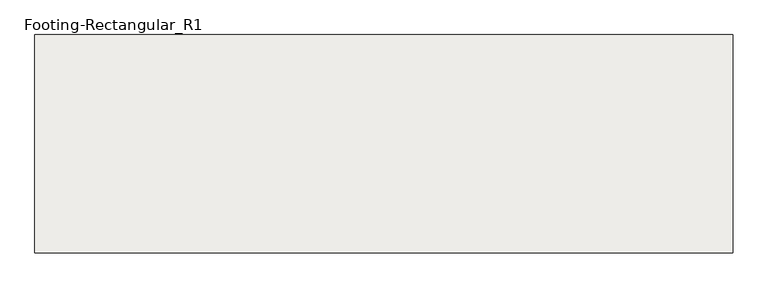
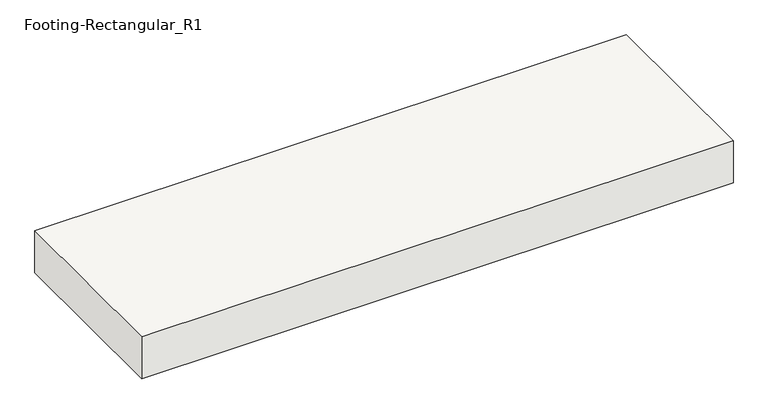
"""IFC4 building model written with IfcOpenShell, lengths in millimetres: slab geometry, Footing-Rectangular_R1 : H_SF_AR_S18_W8000xL2500xT500_Bitumen_F5."""

from ifc_helpers import new_model, si_unit, frame, origin, place, context, project, spatial, polyline, outline, extrude, source, transform, mapped, element, save


def footing_rectangular_r1_282b4f06(model_context):
    return source(origin(), model_context, "Body", "SweptSolid", [
        extrude(outline(polyline([(4000.0, 1250.0), (4000.0, -1250.0), (-4000.0, -1250.0), (-4000.0, 1250.0), (4000.0, 1250.0)])), frame((0.0, 0.0, -600.0), z_axis=(0.0, 0.0, 1.0), x_axis=(1.0, 0.0, 0.0)), (0.0, 0.0, 1.0), 600.0),
    ])


if __name__ == "__main__":
    model = new_model("IFC4")
    model_context = context("Model", 3, world=origin())
    ifc_project = project(units=[si_unit("LENGTHUNIT", "METRE", prefix="MILLI")], contexts=[model_context])
    site = spatial("IfcSite", under=ifc_project)
    building = spatial("IfcBuilding", under=site)
    placement = place(None, origin())
    footing_rectangular_r1_shape = footing_rectangular_r1_282b4f06(model_context)
    element("IfcSlab", 1, ObjectType="Footing-Rectangular_R1 : H_SF_AR_S18_W8000xL2500xT500_Bitumen_F5", at=placement, inside=building, context=model_context, shape_type="MappedRepresentation", body=[
        mapped(footing_rectangular_r1_shape, transform((0.0, 0.0, 0.0), x_axis=(1.0, 0.0, 0.0), y_axis=(0.0, 1.0, 0.0), z_axis=(0.0, 0.0, 1.0))),
    ])
    save(model, "model.ifc")

# Revit data of these elements
# Type "Footing-Rectangular_R1 : H_SF_AR_S18_W8000xL2500xT500_Bitumen_F5"
#   Type Mark = "F5"
#   Top bar = "D25@300"
#   Description = "UG Shallow Foundation"
#   Bottom bar = "D20@300"
#   Width = 8000 mm
#   Length = 2500 mm
#   Foundation Thickness = 600 mm
#   Structural Material [instance default] = none
#   Assembly Code = ""
